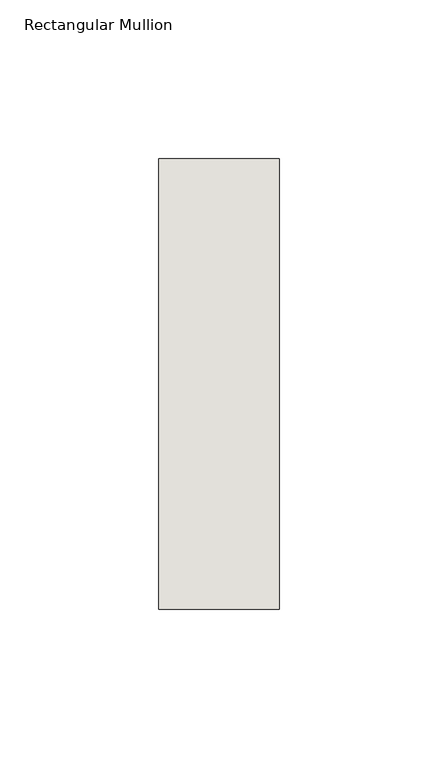
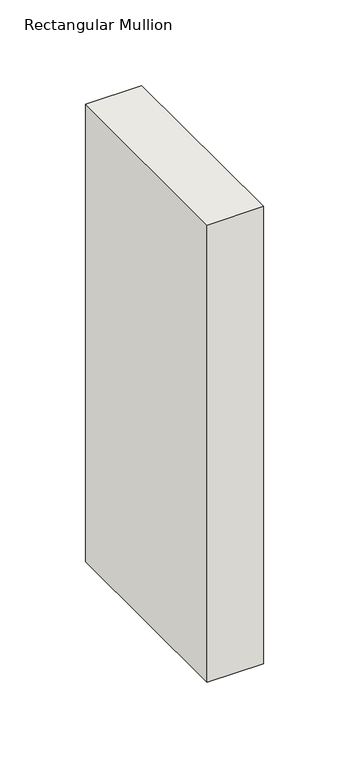
"""IFC4 building model written with IfcOpenShell, lengths in millimetres: wall geometry, Rectangular Mullion : NLRS_21_CWM_hsb-regel 38x142_gen_rsf."""

import ifcopenshell
import ifcopenshell.guid

model = None  # the IFC model being written
_history = None  # IfcOwnerHistory: only IFC2X3 demands one
_inside = {}  # id of a spatial element -> (the spatial element, [elements in it])
_under = {}  # id of a project, library or spatial element -> (it, [spatial elements below it])
_declared = {}  # id of a project -> (the project, [libraries it declares])
_typed = {}  # id of a type object -> (the type object, [elements of that type])
_made_of = {}  # id of a material, layer set ... -> (it, [elements and type objects made of it])


def new_model(schema):
    """Start an empty IFC model of exactly this schema.

    Asked for "IFC4X3", IfcOpenShell would pick the latest addendum, in which some entities
    have other attributes; the version numbers below select the first issue.
    IFC2X3 requires an IfcOwnerHistory on every rooted entity: one is made here for all.
    """
    global model, _history
    if schema == "IFC4X3":
        model = ifcopenshell.file(schema_version=(4, 3, 0, 0))
    else:
        model = ifcopenshell.file(schema=schema)
    _inside.clear()
    _under.clear()
    _declared.clear()
    _typed.clear()
    _made_of.clear()
    _history = None
    if model.schema == "IFC2X3":
        org = make("IfcOrganization", Name="unknown")
        user = make(
            "IfcPersonAndOrganization",
            ThePerson=make("IfcPerson", FamilyName="unknown"),
            TheOrganization=org,
        )
        app = make(
            "IfcApplication",
            ApplicationDeveloper=org,
            Version="unknown",
            ApplicationFullName="unknown",
            ApplicationIdentifier="unknown",
        )
        _history = make(
            "IfcOwnerHistory",
            OwningUser=user,
            OwningApplication=app,
            ChangeAction="ADDED",
            CreationDate=0,
        )
    return model


def make(cls, **values):
    """One entity of the class cls with the attributes given. An attribute that is None is left unset."""
    return model.create_entity(
        cls, **{name: value for name, value in values.items() if value is not None}
    )


def rooted(cls, **values):
    """An entity with a GlobalId (a new one), such as an element, a storey or a relation."""
    return make(cls, GlobalId=ifcopenshell.guid.new(), OwnerHistory=_history, **values)


def si_unit(unit_type, name, prefix=None):
    """IfcSIUnit, for example si_unit("LENGTHUNIT", "METRE", prefix="MILLI")."""
    return make("IfcSIUnit", UnitType=unit_type, Prefix=prefix, Name=name)


def assignment(units):
    """IfcUnitAssignment: the units of a project."""
    return None if units is None else make("IfcUnitAssignment", Units=units)


def point(xyz):
    """IfcCartesianPoint."""
    return None if xyz is None else make("IfcCartesianPoint", Coordinates=xyz)


def direction(xyz):
    """IfcDirection."""
    return None if xyz is None else make("IfcDirection", DirectionRatios=xyz)


def frame(location, z_axis=None, x_axis=None):
    """IfcAxis2Placement3D, a coordinate frame: its origin and axes. An axis left out is left unset."""
    return make(
        "IfcAxis2Placement3D",
        Location=point(location),
        Axis=direction(z_axis),
        RefDirection=direction(x_axis),
    )


def origin():
    """The frame at (0, 0, 0) with its axes left unset."""
    return frame((0.0, 0.0, 0.0))


def place(relative_to, where):
    """IfcLocalPlacement: puts the frame where relative to a parent placement (None: the world)."""
    return make(
        "IfcLocalPlacement", PlacementRelTo=relative_to, RelativePlacement=where
    )


def context(
    kind, dimensions, precision=None, world=None, true_north=None, identifier=None
):
    """IfcGeometricRepresentationContext, for example the 3D "Model" context."""
    return make(
        "IfcGeometricRepresentationContext",
        ContextIdentifier=identifier,
        ContextType=kind,
        CoordinateSpaceDimension=dimensions,
        Precision=precision,
        WorldCoordinateSystem=world,
        TrueNorth=true_north,
    )


def project(units=None, contexts=None):
    """IfcProject with its units and contexts."""
    return rooted(
        "IfcProject",
        Name="project",
        RepresentationContexts=contexts,
        UnitsInContext=assignment(units),
    )


def spatial(cls, under=None, at=None, **own):
    """A site, building, storey or space (cls), placed at a placement, below another one or the project."""
    s = rooted(cls, ObjectPlacement=at, **own)
    if under is not None:
        _under.setdefault(under.id(), (under, []))[1].append(s)
    return s


def polyline(points):
    """IfcPolyline through the points."""
    return make("IfcPolyline", Points=[point(p) for p in points])


def outline(outer, holes=None, kind="AREA"):
    """IfcArbitraryClosedProfileDef: a profile drawn as a closed curve; with holes, ...WithVoids."""
    if holes is None:
        return make("IfcArbitraryClosedProfileDef", ProfileType=kind, OuterCurve=outer)
    return make(
        "IfcArbitraryProfileDefWithVoids",
        ProfileType=kind,
        OuterCurve=outer,
        InnerCurves=holes,
    )


def extrude(swept, where, along, depth):
    """IfcExtrudedAreaSolid: the profile swept, set in the frame where, extruded along a direction by depth."""
    return make(
        "IfcExtrudedAreaSolid",
        SweptArea=swept,
        Position=where,
        ExtrudedDirection=direction(along),
        Depth=depth,
    )


def shape(context_of_items, identifier, shape_type, items):
    """IfcShapeRepresentation: the items that make up one representation, for example the "Body"."""
    return make(
        "IfcShapeRepresentation",
        ContextOfItems=context_of_items,
        RepresentationIdentifier=identifier,
        RepresentationType=shape_type,
        Items=items,
    )


def source(mapping_origin, context_of_items, identifier, shape_type, items):
    """IfcRepresentationMap: a shape defined once, which mapped items show again and again."""
    return make(
        "IfcRepresentationMap",
        MappingOrigin=mapping_origin,
        MappedRepresentation=shape(context_of_items, identifier, shape_type, items),
    )


def transform(
    local_origin,
    x_axis=None,
    y_axis=None,
    z_axis=None,
    scale=None,
    scale2=None,
    scale3=None,
    uniform=True,
):
    """IfcCartesianTransformationOperator3D, or its non-uniform kind. x_axis, y_axis, z_axis: its Axis1, 2, 3."""
    if uniform:
        return make(
            "IfcCartesianTransformationOperator3D",
            Axis1=direction(x_axis),
            Axis2=direction(y_axis),
            LocalOrigin=point(local_origin),
            Scale=scale,
            Axis3=direction(z_axis),
        )
    return make(
        "IfcCartesianTransformationOperator3DnonUniform",
        Axis1=direction(x_axis),
        Axis2=direction(y_axis),
        LocalOrigin=point(local_origin),
        Scale=scale,
        Axis3=direction(z_axis),
        Scale2=scale2,
        Scale3=scale3,
    )


def mapped(mapping_source, mapping_target):
    """IfcMappedItem: shows the shape of a source again, moved by a transform."""
    return make(
        "IfcMappedItem", MappingSource=mapping_source, MappingTarget=mapping_target
    )


def made_of(thing, what):
    """Note that an element or type object is made of a material, layer set ...; save() writes the relation."""
    if what is not None:
        _made_of.setdefault(what.id(), (what, []))[1].append(thing)
    return thing


def element(
    cls,
    number,
    at=None,
    inside=None,
    cuts=None,
    type_object=None,
    material=None,
    context=None,
    identifier="Body",
    shape_type=None,
    held_by="IfcProductDefinitionShape",
    body=None,
    shapes=None,
    **own,
):
    """One element of the class cls, such as IfcWall. Its Tag is "e" and its number.

    at: its placement. inside: the storey or other place that contains it. cuts: it is an
    opening in that element (IfcRelVoidsElement). A single representation is given by context,
    identifier, shape_type and body (its items); several are given by shapes. held_by: the class
    of the entity that holds the representations. save() writes the other relations.
    """
    e = rooted(cls, Tag="e%d" % number, ObjectPlacement=at, **own)
    if body is not None:
        shapes = [shape(context, identifier, shape_type, body)]
    if shapes is not None:
        e.Representation = make(held_by, Representations=shapes)
    if inside is not None:
        _inside.setdefault(inside.id(), (inside, []))[1].append(e)
    if cuts is not None:
        rooted(
            "IfcRelVoidsElement", RelatingBuildingElement=cuts, RelatedOpeningElement=e
        )
    if type_object is not None:
        _typed.setdefault(type_object.id(), (type_object, []))[1].append(e)
    return made_of(e, material)


def aggregate(whole, parts):
    """IfcRelAggregates: a whole, such as a stair, and the parts it consists of."""
    return rooted("IfcRelAggregates", RelatingObject=whole, RelatedObjects=parts)


def save(model, path):
    """Write the relations noted so far, then the file.

    IfcRelAggregates (storeys below a building ...), IfcRelContainedInSpatialStructure (elements
    in a storey), IfcRelDefinesByType, IfcRelAssociatesMaterial and IfcRelDeclares: one each for
    every whole, place, type object, material and project.
    """
    for whole, parts in _under.values():
        aggregate(whole, parts)
    for where, things in _inside.values():
        rooted(
            "IfcRelContainedInSpatialStructure",
            RelatedElements=things,
            RelatingStructure=where,
        )
    for kind, things in _typed.values():
        rooted("IfcRelDefinesByType", RelatedObjects=things, RelatingType=kind)
    for what, things in _made_of.values():
        rooted("IfcRelAssociatesMaterial", RelatedObjects=things, RelatingMaterial=what)
    for by, libraries in _declared.values():
        rooted("IfcRelDeclares", RelatingContext=by, RelatedDefinitions=libraries)
    model.write(path)


def rectangular_mullion_66002bf8(model_context):
    return source(origin(), model_context, "Body", "SweptSolid", [
        extrude(outline(polyline([(-38.0, -71.0), (-38.0, 71.0), (0.0, 71.0), (0.0, -71.0), (-38.0, -71.0)])), frame((0.0, 0.0, -326.0000003), z_axis=(0.0, 0.0, 1.0), x_axis=(1.0, 0.0, 0.0)), (0.0, 0.0, 1.0), 326.0000003),
    ])


if __name__ == "__main__":
    model = new_model("IFC4")
    model_context = context("Model", 3, world=origin())
    ifc_project = project(units=[si_unit("LENGTHUNIT", "METRE", prefix="MILLI")], contexts=[model_context])
    site = spatial("IfcSite", under=ifc_project)
    building = spatial("IfcBuilding", under=site)
    placement = place(None, origin())
    rectangular_mullion_shape = rectangular_mullion_66002bf8(model_context)
    element("IfcWall", 1, ObjectType="Rectangular Mullion : NLRS_21_CWM_hsb-regel 38x142_gen_rsf", at=placement, inside=building, context=model_context, shape_type="MappedRepresentation", body=[
        mapped(rectangular_mullion_shape, transform((0.0, 0.0, 0.0), x_axis=(1.0, 0.0, 0.0), y_axis=(0.0, 1.0, 0.0), z_axis=(0.0, 0.0, 1.0))),
    ])
    save(model, "model.ifc")

# Revit data of these elements
# Type "Rectangular Mullion : NLRS_21_CWM_hsb-regel 38x142_gen_rsf"
#   Type IfcGUID = "07M7mRoiH1CR8m_RSKIwpF"
#   Assembly Code = "21.10"
#   IfcExportAs = "IfcWall"
#   built-in parameter 1007322 = 0.465879 (stored number, unit not read)
#   built-in parameter 1007321 = 0.062336 (stored number, unit not read)
#   built-in parameter 1007320 = 0.062336 (stored number, unit not read)
# Element 1 (IfcWall, "Rectangular Mullion : NLRS_21_CWM_hsb-regel 38x142_gen_rsf")
#   Materials on its faces: "NLRS_i2_hout naaldhout vuren_gen_rsf"
# Materials
#   "NLRS_i2_hout naaldhout vuren_gen_rsf": class "I - Hout", colour RGB 234 199 147, transparency 0, Keynote = "i2", Manufacturer = "Revit Standards Foundation", URL = "www.revitstandards.org", Description = "hout vuren", Cost = 0
